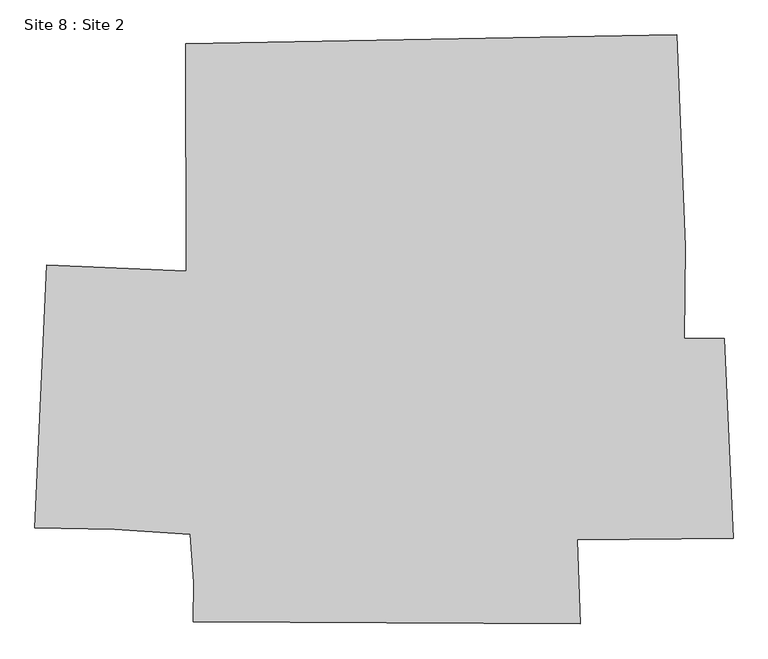
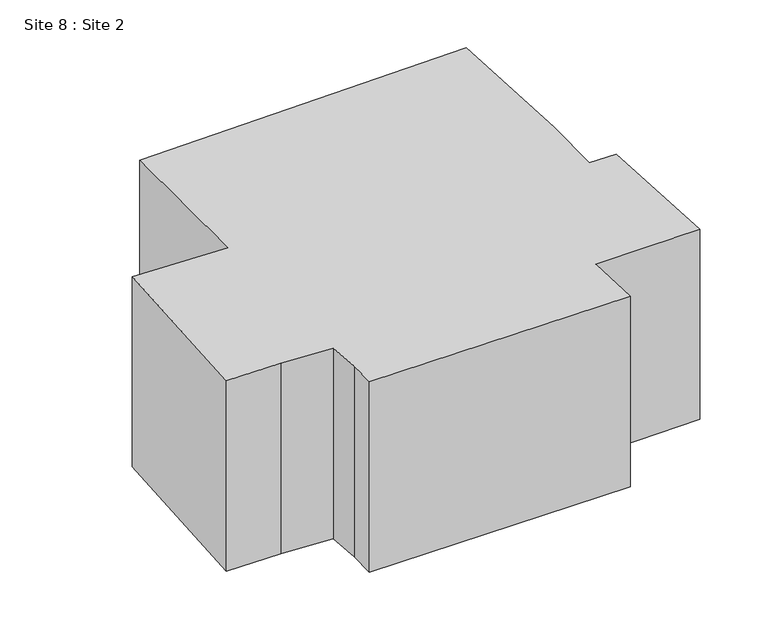
"""IFC4 building model written with IfcOpenShell, lengths in millimetres: geographic element geometry, Site 8 : Site 2."""

from ifc_helpers import new_model, si_unit, frame, origin, place, context, project, spatial, polyline, outline, extrude, source, transform, mapped, element, save


def site_8_site_2_3ba1f17e(model_context):
    return source(origin(), model_context, "Body", "SweptSolid", [
        extrude(outline(polyline([(17136.7272759, 29780.0507186), (18152.6239295, 29765.3331737), (18383.8030411, 24681.5193473), (14420.3487659, 24637.3304383), (14491.0298199, 22502.5290813), (4635.3952714, 22543.7016386), (4650.1124484, 23559.5728954), (4566.1817023, 24780.0901826), (2637.4557041, 24909.6405578), (605.6708625, 24939.075525), (905.9833281, 31640.9246511), (4460.1371995, 31487.8263022), (4442.438596, 37279.8065116), (16943.8128244, 37505.1298127), (17170.576783, 32116.5546092), (17136.7272759, 29780.0507186)])), frame((0.0, 0.0, 266395.2), z_axis=(0.0, 0.0, 1.0), x_axis=(1.0, 0.0, 0.0)), (0.0, 0.0, 1.0), 7620.0),
    ])


if __name__ == "__main__":
    model = new_model("IFC4")
    model_context = context("Model", 3, world=origin())
    ifc_project = project(units=[si_unit("LENGTHUNIT", "METRE", prefix="MILLI")], contexts=[model_context])
    site = spatial("IfcSite", under=ifc_project)
    building = spatial("IfcBuilding", under=site)
    placement = place(None, origin())
    site_8_site_2_shape = site_8_site_2_3ba1f17e(model_context)
    element("IfcGeographicElement", 1, ObjectType="Site 8 : Site 2", at=placement, inside=building, context=model_context, shape_type="MappedRepresentation", body=[
        mapped(site_8_site_2_shape, transform((0.0, 0.0, 0.0), x_axis=(1.0, 0.0, 0.0), y_axis=(0.0, 1.0, 0.0), z_axis=(0.0, 0.0, 1.0))),
    ])
    save(model, "model.ifc")

# Revit data of these elements
# Element 1 (IfcGeographicElement, "Site 8 : Site 2")
#   Materials on its faces: "EXISTING BUILDING"
# Materials
#   "EXISTING BUILDING": class "Generic", colour RGB 120 120 120, transparency 0, Cost = 0
